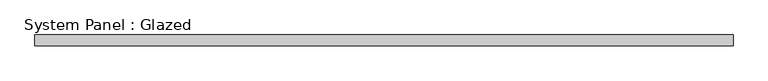
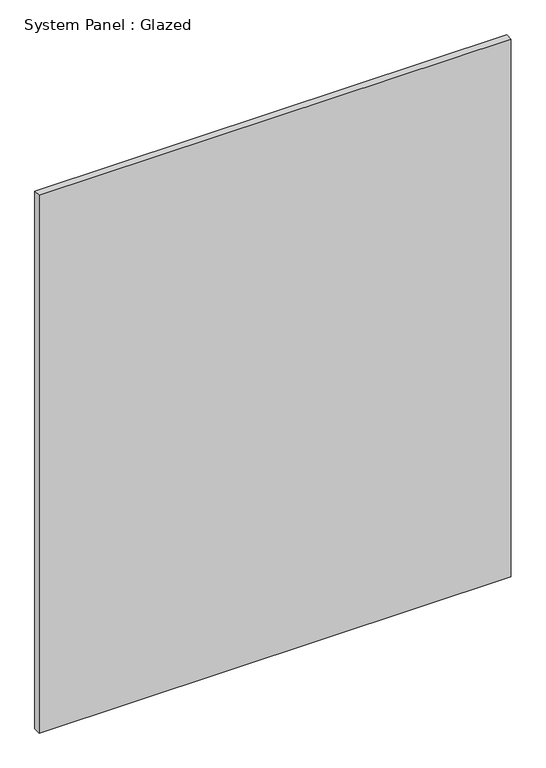
"""IFC4 building model written with IfcOpenShell, lengths in millimetres: plate geometry, System Panel : Glazed."""

import ifcopenshell
import ifcopenshell.guid

model = None  # the IFC model being written
_history = None  # IfcOwnerHistory: only IFC2X3 demands one
_inside = {}  # id of a spatial element -> (the spatial element, [elements in it])
_under = {}  # id of a project, library or spatial element -> (it, [spatial elements below it])
_declared = {}  # id of a project -> (the project, [libraries it declares])
_typed = {}  # id of a type object -> (the type object, [elements of that type])
_made_of = {}  # id of a material, layer set ... -> (it, [elements and type objects made of it])


def new_model(schema):
    """Start an empty IFC model of exactly this schema.

    Asked for "IFC4X3", IfcOpenShell would pick the latest addendum, in which some entities
    have other attributes; the version numbers below select the first issue.
    IFC2X3 requires an IfcOwnerHistory on every rooted entity: one is made here for all.
    """
    global model, _history
    if schema == "IFC4X3":
        model = ifcopenshell.file(schema_version=(4, 3, 0, 0))
    else:
        model = ifcopenshell.file(schema=schema)
    _inside.clear()
    _under.clear()
    _declared.clear()
    _typed.clear()
    _made_of.clear()
    _history = None
    if model.schema == "IFC2X3":
        org = make("IfcOrganization", Name="unknown")
        user = make(
            "IfcPersonAndOrganization",
            ThePerson=make("IfcPerson", FamilyName="unknown"),
            TheOrganization=org,
        )
        app = make(
            "IfcApplication",
            ApplicationDeveloper=org,
            Version="unknown",
            ApplicationFullName="unknown",
            ApplicationIdentifier="unknown",
        )
        _history = make(
            "IfcOwnerHistory",
            OwningUser=user,
            OwningApplication=app,
            ChangeAction="ADDED",
            CreationDate=0,
        )
    return model


def make(cls, **values):
    """One entity of the class cls with the attributes given. An attribute that is None is left unset."""
    return model.create_entity(
        cls, **{name: value for name, value in values.items() if value is not None}
    )


def rooted(cls, **values):
    """An entity with a GlobalId (a new one), such as an element, a storey or a relation."""
    return make(cls, GlobalId=ifcopenshell.guid.new(), OwnerHistory=_history, **values)


def si_unit(unit_type, name, prefix=None):
    """IfcSIUnit, for example si_unit("LENGTHUNIT", "METRE", prefix="MILLI")."""
    return make("IfcSIUnit", UnitType=unit_type, Prefix=prefix, Name=name)


def assignment(units):
    """IfcUnitAssignment: the units of a project."""
    return None if units is None else make("IfcUnitAssignment", Units=units)


def point(xyz):
    """IfcCartesianPoint."""
    return None if xyz is None else make("IfcCartesianPoint", Coordinates=xyz)


def direction(xyz):
    """IfcDirection."""
    return None if xyz is None else make("IfcDirection", DirectionRatios=xyz)


def frame(location, z_axis=None, x_axis=None):
    """IfcAxis2Placement3D, a coordinate frame: its origin and axes. An axis left out is left unset."""
    return make(
        "IfcAxis2Placement3D",
        Location=point(location),
        Axis=direction(z_axis),
        RefDirection=direction(x_axis),
    )


def origin():
    """The frame at (0, 0, 0) with its axes left unset."""
    return frame((0.0, 0.0, 0.0))


def origin_with_axes():
    """The frame at (0, 0, 0) with the z axis (0, 0, 1) and the x axis (1, 0, 0) written out."""
    return frame((0.0, 0.0, 0.0), z_axis=(0.0, 0.0, 1.0), x_axis=(1.0, 0.0, 0.0))


def place(relative_to, where):
    """IfcLocalPlacement: puts the frame where relative to a parent placement (None: the world)."""
    return make(
        "IfcLocalPlacement", PlacementRelTo=relative_to, RelativePlacement=where
    )


def context(
    kind, dimensions, precision=None, world=None, true_north=None, identifier=None
):
    """IfcGeometricRepresentationContext, for example the 3D "Model" context."""
    return make(
        "IfcGeometricRepresentationContext",
        ContextIdentifier=identifier,
        ContextType=kind,
        CoordinateSpaceDimension=dimensions,
        Precision=precision,
        WorldCoordinateSystem=world,
        TrueNorth=true_north,
    )


def project(units=None, contexts=None):
    """IfcProject with its units and contexts."""
    return rooted(
        "IfcProject",
        Name="project",
        RepresentationContexts=contexts,
        UnitsInContext=assignment(units),
    )


def spatial(cls, under=None, at=None, **own):
    """A site, building, storey or space (cls), placed at a placement, below another one or the project."""
    s = rooted(cls, ObjectPlacement=at, **own)
    if under is not None:
        _under.setdefault(under.id(), (under, []))[1].append(s)
    return s


def polyline(points):
    """IfcPolyline through the points."""
    return make("IfcPolyline", Points=[point(p) for p in points])


def outline(outer, holes=None, kind="AREA"):
    """IfcArbitraryClosedProfileDef: a profile drawn as a closed curve; with holes, ...WithVoids."""
    if holes is None:
        return make("IfcArbitraryClosedProfileDef", ProfileType=kind, OuterCurve=outer)
    return make(
        "IfcArbitraryProfileDefWithVoids",
        ProfileType=kind,
        OuterCurve=outer,
        InnerCurves=holes,
    )


def extrude(swept, where, along, depth):
    """IfcExtrudedAreaSolid: the profile swept, set in the frame where, extruded along a direction by depth."""
    return make(
        "IfcExtrudedAreaSolid",
        SweptArea=swept,
        Position=where,
        ExtrudedDirection=direction(along),
        Depth=depth,
    )


def shape(context_of_items, identifier, shape_type, items):
    """IfcShapeRepresentation: the items that make up one representation, for example the "Body"."""
    return make(
        "IfcShapeRepresentation",
        ContextOfItems=context_of_items,
        RepresentationIdentifier=identifier,
        RepresentationType=shape_type,
        Items=items,
    )


def source(mapping_origin, context_of_items, identifier, shape_type, items):
    """IfcRepresentationMap: a shape defined once, which mapped items show again and again."""
    return make(
        "IfcRepresentationMap",
        MappingOrigin=mapping_origin,
        MappedRepresentation=shape(context_of_items, identifier, shape_type, items),
    )


def transform(
    local_origin,
    x_axis=None,
    y_axis=None,
    z_axis=None,
    scale=None,
    scale2=None,
    scale3=None,
    uniform=True,
):
    """IfcCartesianTransformationOperator3D, or its non-uniform kind. x_axis, y_axis, z_axis: its Axis1, 2, 3."""
    if uniform:
        return make(
            "IfcCartesianTransformationOperator3D",
            Axis1=direction(x_axis),
            Axis2=direction(y_axis),
            LocalOrigin=point(local_origin),
            Scale=scale,
            Axis3=direction(z_axis),
        )
    return make(
        "IfcCartesianTransformationOperator3DnonUniform",
        Axis1=direction(x_axis),
        Axis2=direction(y_axis),
        LocalOrigin=point(local_origin),
        Scale=scale,
        Axis3=direction(z_axis),
        Scale2=scale2,
        Scale3=scale3,
    )


def mapped(mapping_source, mapping_target):
    """IfcMappedItem: shows the shape of a source again, moved by a transform."""
    return make(
        "IfcMappedItem", MappingSource=mapping_source, MappingTarget=mapping_target
    )


def made_of(thing, what):
    """Note that an element or type object is made of a material, layer set ...; save() writes the relation."""
    if what is not None:
        _made_of.setdefault(what.id(), (what, []))[1].append(thing)
    return thing


def element(
    cls,
    number,
    at=None,
    inside=None,
    cuts=None,
    type_object=None,
    material=None,
    context=None,
    identifier="Body",
    shape_type=None,
    held_by="IfcProductDefinitionShape",
    body=None,
    shapes=None,
    **own,
):
    """One element of the class cls, such as IfcWall. Its Tag is "e" and its number.

    at: its placement. inside: the storey or other place that contains it. cuts: it is an
    opening in that element (IfcRelVoidsElement). A single representation is given by context,
    identifier, shape_type and body (its items); several are given by shapes. held_by: the class
    of the entity that holds the representations. save() writes the other relations.
    """
    e = rooted(cls, Tag="e%d" % number, ObjectPlacement=at, **own)
    if body is not None:
        shapes = [shape(context, identifier, shape_type, body)]
    if shapes is not None:
        e.Representation = make(held_by, Representations=shapes)
    if inside is not None:
        _inside.setdefault(inside.id(), (inside, []))[1].append(e)
    if cuts is not None:
        rooted(
            "IfcRelVoidsElement", RelatingBuildingElement=cuts, RelatedOpeningElement=e
        )
    if type_object is not None:
        _typed.setdefault(type_object.id(), (type_object, []))[1].append(e)
    return made_of(e, material)


def aggregate(whole, parts):
    """IfcRelAggregates: a whole, such as a stair, and the parts it consists of."""
    return rooted("IfcRelAggregates", RelatingObject=whole, RelatedObjects=parts)


def save(model, path):
    """Write the relations noted so far, then the file.

    IfcRelAggregates (storeys below a building ...), IfcRelContainedInSpatialStructure (elements
    in a storey), IfcRelDefinesByType, IfcRelAssociatesMaterial and IfcRelDeclares: one each for
    every whole, place, type object, material and project.
    """
    for whole, parts in _under.values():
        aggregate(whole, parts)
    for where, things in _inside.values():
        rooted(
            "IfcRelContainedInSpatialStructure",
            RelatedElements=things,
            RelatingStructure=where,
        )
    for kind, things in _typed.values():
        rooted("IfcRelDefinesByType", RelatedObjects=things, RelatingType=kind)
    for what, things in _made_of.values():
        rooted("IfcRelAssociatesMaterial", RelatedObjects=things, RelatingMaterial=what)
    for by, libraries in _declared.values():
        rooted("IfcRelDeclares", RelatingContext=by, RelatedDefinitions=libraries)
    model.write(path)


def system_panel_glazed_da9c9e0f(model_context):
    return source(origin(), model_context, "Body", "SweptSolid", [
        extrude(outline(polyline([(810.0, 24.5), (-810.0, 24.5), (-810.0, 49.5), (810.0, 49.5), (810.0, 24.5)])), origin_with_axes(), (0.0, 0.0, 1.0), 1950.0),
    ])


if __name__ == "__main__":
    model = new_model("IFC4")
    model_context = context("Model", 3, world=origin())
    ifc_project = project(units=[si_unit("LENGTHUNIT", "METRE", prefix="MILLI")], contexts=[model_context])
    site = spatial("IfcSite", under=ifc_project)
    building = spatial("IfcBuilding", under=site)
    placement = place(None, origin())
    system_panel_glazed_shape = system_panel_glazed_da9c9e0f(model_context)
    element("IfcPlate", 1, ObjectType="System Panel : Glazed", at=placement, inside=building, context=model_context, shape_type="MappedRepresentation", body=[
        mapped(system_panel_glazed_shape, transform((0.0, 0.0, 0.0), x_axis=(1.0, 0.0, 0.0), y_axis=(0.0, 1.0, 0.0), z_axis=(0.0, 0.0, 1.0))),
    ])
    save(model, "model.ifc")

# Revit data of these elements
# Element 1 (IfcPlate, "System Panel : Glazed")
#   Materials on its faces: "Glass"
# Materials
#   "Glass": class "Glass", colour RGB 0 128 192, transparency 0.9
